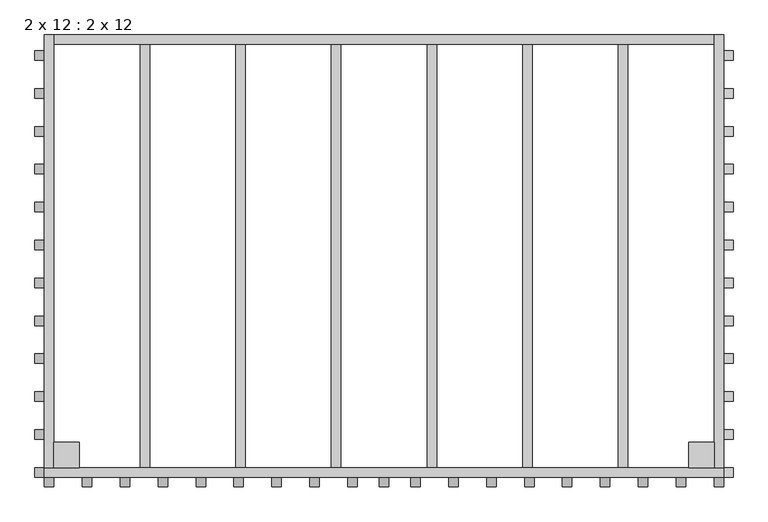
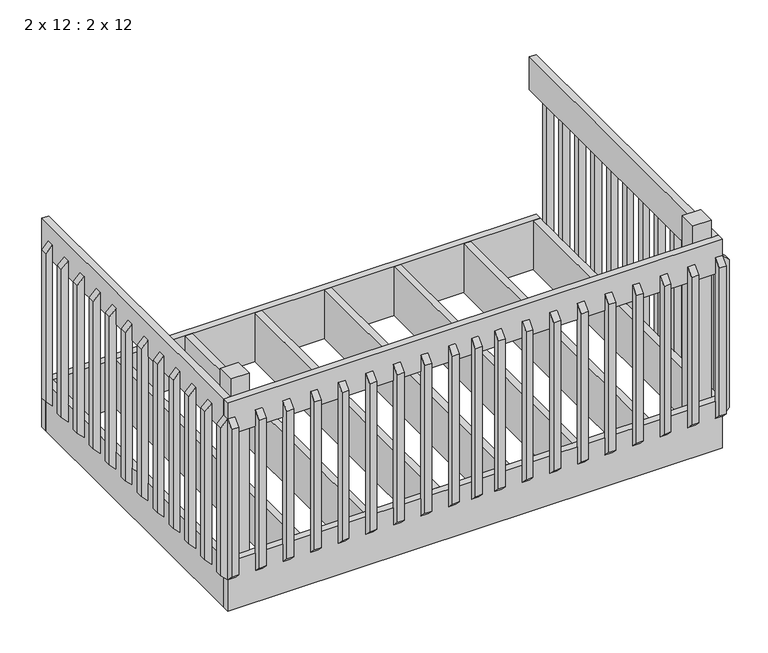
"""IFC4 building model written with IfcOpenShell, lengths in millimetres: proxy geometry, 2 x 12 : 2 x 12."""

from ifc_helpers import new_model, si_unit, frame, origin, place, context, project, spatial, polyline, outline, extrude, source, transform, mapped, element, save


def proxy_2_x_12_2_x_12_a4ed22fe(model_context):
    return source(origin(), model_context, "Body", "SweptSolid", [
        extrude(outline(polyline([(-24301.8830088, 3282.95), (-24339.9830088, 3321.05), (-24339.9830088, 4184.65), (-24301.8830088, 4222.75), (-24301.8830088, 3282.95)])), frame((31168.6652986, 0.0, 0.0), z_axis=(1.0, 0.0, 0.0), x_axis=(0.0, 1.0, 0.0)), (0.0, 0.0, 1.0), 38.1),
        extrude(outline(polyline([(-24301.8830088, 3282.95), (-24339.9830088, 3321.05), (-24339.9830088, 4184.65), (-24301.8830088, 4222.75), (-24301.8830088, 3282.95)])), frame((31295.6652986, 0.0, 0.0), z_axis=(1.0, 0.0, 0.0), x_axis=(0.0, 1.0, 0.0)), (0.0, 0.0, 1.0), 38.1),
        extrude(outline(polyline([(-24301.8830088, 3282.95), (-24339.9830088, 3321.05), (-24339.9830088, 4184.65), (-24301.8830088, 4222.75), (-24301.8830088, 3282.95)])), frame((31448.0652986, 0.0, 0.0), z_axis=(1.0, 0.0, 0.0), x_axis=(0.0, 1.0, 0.0)), (0.0, 0.0, 1.0), 38.1),
        extrude(outline(polyline([(-24301.8830088, 3282.95), (-24339.9830088, 3321.05), (-24339.9830088, 4184.65), (-24301.8830088, 4222.75), (-24301.8830088, 3282.95)])), frame((31600.4652986, 0.0, 0.0), z_axis=(1.0, 0.0, 0.0), x_axis=(0.0, 1.0, 0.0)), (0.0, 0.0, 1.0), 38.1),
        extrude(outline(polyline([(-24301.8830088, 3282.95), (-24339.9830088, 3321.05), (-24339.9830088, 4184.65), (-24301.8830088, 4222.75), (-24301.8830088, 3282.95)])), frame((31752.8652986, 0.0, 0.0), z_axis=(1.0, 0.0, 0.0), x_axis=(0.0, 1.0, 0.0)), (0.0, 0.0, 1.0), 38.1),
        extrude(outline(polyline([(-24301.8830088, 3282.95), (-24339.9830088, 3321.05), (-24339.9830088, 4184.65), (-24301.8830088, 4222.75), (-24301.8830088, 3282.95)])), frame((31905.2652986, 0.0, 0.0), z_axis=(1.0, 0.0, 0.0), x_axis=(0.0, 1.0, 0.0)), (0.0, 0.0, 1.0), 38.1),
        extrude(outline(polyline([(-24301.8830088, 3282.95), (-24339.9830088, 3321.05), (-24339.9830088, 4184.65), (-24301.8830088, 4222.75), (-24301.8830088, 3282.95)])), frame((32057.6652986, 0.0, 0.0), z_axis=(1.0, 0.0, 0.0), x_axis=(0.0, 1.0, 0.0)), (0.0, 0.0, 1.0), 38.1),
        extrude(outline(polyline([(-24301.8830088, 3282.95), (-24339.9830088, 3321.05), (-24339.9830088, 4184.65), (-24301.8830088, 4222.75), (-24301.8830088, 3282.95)])), frame((32210.0652986, 0.0, 0.0), z_axis=(1.0, 0.0, 0.0), x_axis=(0.0, 1.0, 0.0)), (0.0, 0.0, 1.0), 38.1),
        extrude(outline(polyline([(-24301.8830088, 3282.95), (-24339.9830088, 3321.05), (-24339.9830088, 4184.65), (-24301.8830088, 4222.75), (-24301.8830088, 3282.95)])), frame((32362.4652986, 0.0, 0.0), z_axis=(1.0, 0.0, 0.0), x_axis=(0.0, 1.0, 0.0)), (0.0, 0.0, 1.0), 38.1),
        extrude(outline(polyline([(-24301.8830088, 3282.95), (-24339.9830088, 3321.05), (-24339.9830088, 4184.65), (-24301.8830088, 4222.75), (-24301.8830088, 3282.95)])), frame((32514.8652986, 0.0, 0.0), z_axis=(1.0, 0.0, 0.0), x_axis=(0.0, 1.0, 0.0)), (0.0, 0.0, 1.0), 38.1),
        extrude(outline(polyline([(-24301.8830088, 3282.95), (-24339.9830088, 3321.05), (-24339.9830088, 4184.65), (-24301.8830088, 4222.75), (-24301.8830088, 3282.95)])), frame((29822.4652986, 0.0, 0.0), z_axis=(1.0, 0.0, 0.0), x_axis=(0.0, 1.0, 0.0)), (0.0, 0.0, 1.0), 38.1),
        extrude(outline(polyline([(-24301.8830088, 3282.95), (-24339.9830088, 3321.05), (-24339.9830088, 4184.65), (-24301.8830088, 4222.75), (-24301.8830088, 3282.95)])), frame((29974.8652986, 0.0, 0.0), z_axis=(1.0, 0.0, 0.0), x_axis=(0.0, 1.0, 0.0)), (0.0, 0.0, 1.0), 38.1),
        extrude(outline(polyline([(-24301.8830088, 3282.95), (-24339.9830088, 3321.05), (-24339.9830088, 4184.65), (-24301.8830088, 4222.75), (-24301.8830088, 3282.95)])), frame((30127.2652986, 0.0, 0.0), z_axis=(1.0, 0.0, 0.0), x_axis=(0.0, 1.0, 0.0)), (0.0, 0.0, 1.0), 38.1),
        extrude(outline(polyline([(-24301.8830088, 3282.95), (-24339.9830088, 3321.05), (-24339.9830088, 4184.65), (-24301.8830088, 4222.75), (-24301.8830088, 3282.95)])), frame((30279.6652986, 0.0, 0.0), z_axis=(1.0, 0.0, 0.0), x_axis=(0.0, 1.0, 0.0)), (0.0, 0.0, 1.0), 38.1),
        extrude(outline(polyline([(-24301.8830088, 3282.95), (-24339.9830088, 3321.05), (-24339.9830088, 4184.65), (-24301.8830088, 4222.75), (-24301.8830088, 3282.95)])), frame((30432.0652986, 0.0, 0.0), z_axis=(1.0, 0.0, 0.0), x_axis=(0.0, 1.0, 0.0)), (0.0, 0.0, 1.0), 38.1),
        extrude(outline(polyline([(-24301.8830088, 3282.95), (-24339.9830088, 3321.05), (-24339.9830088, 4184.65), (-24301.8830088, 4222.75), (-24301.8830088, 3282.95)])), frame((30584.4652986, 0.0, 0.0), z_axis=(1.0, 0.0, 0.0), x_axis=(0.0, 1.0, 0.0)), (0.0, 0.0, 1.0), 38.1),
        extrude(outline(polyline([(-24301.8830088, 3282.95), (-24339.9830088, 3321.05), (-24339.9830088, 4184.65), (-24301.8830088, 4222.75), (-24301.8830088, 3282.95)])), frame((30736.8652986, 0.0, 0.0), z_axis=(1.0, 0.0, 0.0), x_axis=(0.0, 1.0, 0.0)), (0.0, 0.0, 1.0), 38.1),
        extrude(outline(polyline([(-24301.8830088, 3282.95), (-24339.9830088, 3321.05), (-24339.9830088, 4184.65), (-24301.8830088, 4222.75), (-24301.8830088, 3282.95)])), frame((30889.2652986, 0.0, 0.0), z_axis=(1.0, 0.0, 0.0), x_axis=(0.0, 1.0, 0.0)), (0.0, 0.0, 1.0), 38.1),
        extrude(outline(polyline([(-24301.8830088, 3282.95), (-24339.9830088, 3321.05), (-24339.9830088, 4184.65), (-24301.8830088, 4222.75), (-24301.8830088, 3282.95)])), frame((31041.6652986, 0.0, 0.0), z_axis=(1.0, 0.0, 0.0), x_axis=(0.0, 1.0, 0.0)), (0.0, 0.0, 1.0), 38.1),
        extrude(outline(polyline([(3282.95, 29822.4652986), (4222.75, 29822.4652986), (4184.65, 29784.3652986), (3321.05, 29784.3652986), (3282.95, 29822.4652986)])), frame((0.0, -22625.4830088, 0.0), z_axis=(0.0, 1.0, 0.0), x_axis=(0.0, 0.0, 1.0)), (0.0, 0.0, 1.0), 38.1),
        extrude(outline(polyline([(3282.95, 29822.4652986), (4222.75, 29822.4652986), (4184.65, 29784.3652986), (3321.05, 29784.3652986), (3282.95, 29822.4652986)])), frame((0.0, -22777.8830088, 0.0), z_axis=(0.0, 1.0, 0.0), x_axis=(0.0, 0.0, 1.0)), (0.0, 0.0, 1.0), 38.1),
        extrude(outline(polyline([(3282.95, 29822.4652986), (4222.75, 29822.4652986), (4184.65, 29784.3652986), (3321.05, 29784.3652986), (3282.95, 29822.4652986)])), frame((0.0, -22930.2830088, 0.0), z_axis=(0.0, 1.0, 0.0), x_axis=(0.0, 0.0, 1.0)), (0.0, 0.0, 1.0), 38.1),
        extrude(outline(polyline([(3282.95, 29822.4652986), (4222.75, 29822.4652986), (4184.65, 29784.3652986), (3321.05, 29784.3652986), (3282.95, 29822.4652986)])), frame((0.0, -23082.6830088, 0.0), z_axis=(0.0, 1.0, 0.0), x_axis=(0.0, 0.0, 1.0)), (0.0, 0.0, 1.0), 38.1),
        extrude(outline(polyline([(3282.95, 29822.4652986), (4222.75, 29822.4652986), (4184.65, 29784.3652986), (3321.05, 29784.3652986), (3282.95, 29822.4652986)])), frame((0.0, -23235.0830088, 0.0), z_axis=(0.0, 1.0, 0.0), x_axis=(0.0, 0.0, 1.0)), (0.0, 0.0, 1.0), 38.1),
        extrude(outline(polyline([(3282.95, 29822.4652986), (4222.75, 29822.4652986), (4184.65, 29784.3652986), (3321.05, 29784.3652986), (3282.95, 29822.4652986)])), frame((0.0, -23387.4830088, 0.0), z_axis=(0.0, 1.0, 0.0), x_axis=(0.0, 0.0, 1.0)), (0.0, 0.0, 1.0), 38.1),
        extrude(outline(polyline([(3282.95, 29822.4652986), (4222.75, 29822.4652986), (4184.65, 29784.3652986), (3321.05, 29784.3652986), (3282.95, 29822.4652986)])), frame((0.0, -23539.8830088, 0.0), z_axis=(0.0, 1.0, 0.0), x_axis=(0.0, 0.0, 1.0)), (0.0, 0.0, 1.0), 38.1),
        extrude(outline(polyline([(3282.95, 29822.4652986), (4222.75, 29822.4652986), (4184.65, 29784.3652986), (3321.05, 29784.3652986), (3282.95, 29822.4652986)])), frame((0.0, -23692.2830088, 0.0), z_axis=(0.0, 1.0, 0.0), x_axis=(0.0, 0.0, 1.0)), (0.0, 0.0, 1.0), 38.1),
        extrude(outline(polyline([(3282.95, 29822.4652986), (4222.75, 29822.4652986), (4184.65, 29784.3652986), (3321.05, 29784.3652986), (3282.95, 29822.4652986)])), frame((0.0, -23844.6830088, 0.0), z_axis=(0.0, 1.0, 0.0), x_axis=(0.0, 0.0, 1.0)), (0.0, 0.0, 1.0), 38.1),
        extrude(outline(polyline([(3282.95, 29822.4652986), (4222.75, 29822.4652986), (4184.65, 29784.3652986), (3321.05, 29784.3652986), (3282.95, 29822.4652986)])), frame((0.0, -23997.0830088, 0.0), z_axis=(0.0, 1.0, 0.0), x_axis=(0.0, 0.0, 1.0)), (0.0, 0.0, 1.0), 38.1),
        extrude(outline(polyline([(3282.95, 29822.4652986), (4222.75, 29822.4652986), (4184.65, 29784.3652986), (3321.05, 29784.3652986), (3282.95, 29822.4652986)])), frame((0.0, -24149.4830088, 0.0), z_axis=(0.0, 1.0, 0.0), x_axis=(0.0, 0.0, 1.0)), (0.0, 0.0, 1.0), 38.1),
        extrude(outline(polyline([(3282.95, 29822.4652986), (4222.75, 29822.4652986), (4184.65, 29784.3652986), (3321.05, 29784.3652986), (3282.95, 29822.4652986)])), frame((0.0, -24301.8830088, 0.0), z_axis=(0.0, 1.0, 0.0), x_axis=(0.0, 0.0, 1.0)), (0.0, 0.0, 1.0), 38.1),
        extrude(outline(polyline([(3282.95, 32552.9652986), (3321.05, 32591.0652986), (4184.65, 32591.0652986), (4222.75, 32552.9652986), (3282.95, 32552.9652986)])), frame((0.0, -22625.4830088, 0.0), z_axis=(0.0, 1.0, 0.0), x_axis=(0.0, 0.0, 1.0)), (0.0, 0.0, 1.0), 38.1),
        extrude(outline(polyline([(3282.95, 32552.9652986), (3321.05, 32591.0652986), (4184.65, 32591.0652986), (4222.75, 32552.9652986), (3282.95, 32552.9652986)])), frame((0.0, -22777.8830088, 0.0), z_axis=(0.0, 1.0, 0.0), x_axis=(0.0, 0.0, 1.0)), (0.0, 0.0, 1.0), 38.1),
        extrude(outline(polyline([(3282.95, 32552.9652986), (3321.05, 32591.0652986), (4184.65, 32591.0652986), (4222.75, 32552.9652986), (3282.95, 32552.9652986)])), frame((0.0, -22930.2830088, 0.0), z_axis=(0.0, 1.0, 0.0), x_axis=(0.0, 0.0, 1.0)), (0.0, 0.0, 1.0), 38.1),
        extrude(outline(polyline([(3282.95, 32552.9652986), (3321.05, 32591.0652986), (4184.65, 32591.0652986), (4222.75, 32552.9652986), (3282.95, 32552.9652986)])), frame((0.0, -23082.6830088, 0.0), z_axis=(0.0, 1.0, 0.0), x_axis=(0.0, 0.0, 1.0)), (0.0, 0.0, 1.0), 38.1),
        extrude(outline(polyline([(3282.95, 32552.9652986), (3321.05, 32591.0652986), (4184.65, 32591.0652986), (4222.75, 32552.9652986), (3282.95, 32552.9652986)])), frame((0.0, -23235.0830088, 0.0), z_axis=(0.0, 1.0, 0.0), x_axis=(0.0, 0.0, 1.0)), (0.0, 0.0, 1.0), 38.1),
        extrude(outline(polyline([(3282.95, 32552.9652986), (3321.05, 32591.0652986), (4184.65, 32591.0652986), (4222.75, 32552.9652986), (3282.95, 32552.9652986)])), frame((0.0, -23387.4830088, 0.0), z_axis=(0.0, 1.0, 0.0), x_axis=(0.0, 0.0, 1.0)), (0.0, 0.0, 1.0), 38.1),
        extrude(outline(polyline([(3282.95, 32552.9652986), (3321.05, 32591.0652986), (4184.65, 32591.0652986), (4222.75, 32552.9652986), (3282.95, 32552.9652986)])), frame((0.0, -23539.8830088, 0.0), z_axis=(0.0, 1.0, 0.0), x_axis=(0.0, 0.0, 1.0)), (0.0, 0.0, 1.0), 38.1),
        extrude(outline(polyline([(3282.95, 32552.9652986), (3321.05, 32591.0652986), (4184.65, 32591.0652986), (4222.75, 32552.9652986), (3282.95, 32552.9652986)])), frame((0.0, -23692.2830088, 0.0), z_axis=(0.0, 1.0, 0.0), x_axis=(0.0, 0.0, 1.0)), (0.0, 0.0, 1.0), 38.1),
        extrude(outline(polyline([(3282.95, 32552.9652986), (3321.05, 32591.0652986), (4184.65, 32591.0652986), (4222.75, 32552.9652986), (3282.95, 32552.9652986)])), frame((0.0, -23844.6830088, 0.0), z_axis=(0.0, 1.0, 0.0), x_axis=(0.0, 0.0, 1.0)), (0.0, 0.0, 1.0), 38.1),
        extrude(outline(polyline([(3282.95, 32552.9652986), (3321.05, 32591.0652986), (4184.65, 32591.0652986), (4222.75, 32552.9652986), (3282.95, 32552.9652986)])), frame((0.0, -23997.0830088, 0.0), z_axis=(0.0, 1.0, 0.0), x_axis=(0.0, 0.0, 1.0)), (0.0, 0.0, 1.0), 38.1),
        extrude(outline(polyline([(3282.95, 32552.9652986), (3321.05, 32591.0652986), (4184.65, 32591.0652986), (4222.75, 32552.9652986), (3282.95, 32552.9652986)])), frame((0.0, -24149.4830088, 0.0), z_axis=(0.0, 1.0, 0.0), x_axis=(0.0, 0.0, 1.0)), (0.0, 0.0, 1.0), 38.1),
        extrude(outline(polyline([(3282.95, 32552.9652986), (3321.05, 32591.0652986), (4184.65, 32591.0652986), (4222.75, 32552.9652986), (3282.95, 32552.9652986)])), frame((0.0, -24301.8830088, 0.0), z_axis=(0.0, 1.0, 0.0), x_axis=(0.0, 0.0, 1.0)), (0.0, 0.0, 1.0), 38.1),
        extrude(outline(polyline([(29860.5652986, -24263.7830088), (29822.4652986, -24263.7830088), (29822.4652986, -22523.8830088), (29860.5652986, -22523.8830088), (29860.5652986, -24263.7830088)])), frame((0.0, 0.0, 4127.5), z_axis=(0.0, 0.0, 1.0), x_axis=(1.0, 0.0, 0.0)), (0.0, 0.0, 1.0), 190.5),
        extrude(outline(polyline([(32552.9652986, -24263.7830088), (32514.8652986, -24263.7830088), (32514.8652986, -22523.8830088), (32552.9652986, -22523.8830088), (32552.9652986, -24263.7830088)])), frame((0.0, 0.0, 4127.5), z_axis=(0.0, 0.0, 1.0), x_axis=(1.0, 0.0, 0.0)), (0.0, 0.0, 1.0), 190.5),
        extrude(outline(polyline([(32552.9652986, -24263.7830088), (32552.9652986, -24301.8830088), (29822.4652986, -24301.8830088), (29822.4652986, -24263.7830088), (32552.9652986, -24263.7830088)])), frame((0.0, 0.0, 4127.5), z_axis=(0.0, 0.0, 1.0), x_axis=(1.0, 0.0, 0.0)), (0.0, 0.0, 1.0), 190.5),
        extrude(outline(polyline([(32514.8652986, -24162.1830088), (32514.8652986, -24263.7830088), (32413.2652986, -24263.7830088), (32413.2652986, -24162.1830088), (32514.8652986, -24162.1830088)])), frame((0.0, 0.0, 3098.8), z_axis=(0.0, 0.0, 1.0), x_axis=(1.0, 0.0, 0.0)), (0.0, 0.0, 1.0), 1320.8),
        extrude(outline(polyline([(29962.1652986, -24162.1830088), (29962.1652986, -24263.7830088), (29860.5652986, -24263.7830088), (29860.5652986, -24162.1830088), (29962.1652986, -24162.1830088)])), frame((0.0, 0.0, 3098.8), z_axis=(0.0, 0.0, 1.0), x_axis=(1.0, 0.0, 0.0)), (0.0, 0.0, 1.0), 1320.8),
        extrude(outline(polyline([(32552.9652986, -22523.8830088), (32552.9652986, -22561.9830088), (29822.4652986, -22561.9830088), (29822.4652986, -22523.8830088), (32552.9652986, -22523.8830088)])), frame((0.0, 0.0, 3098.8), z_axis=(0.0, 0.0, 1.0), x_axis=(1.0, 0.0, 0.0)), (0.0, 0.0, 1.0), 285.75),
        extrude(outline(polyline([(32552.9652986, -24263.7830088), (32552.9652986, -24301.8830088), (29822.4652986, -24301.8830088), (29822.4652986, -24263.7830088), (32552.9652986, -24263.7830088)])), frame((0.0, 0.0, 3098.8), z_axis=(0.0, 0.0, 1.0), x_axis=(1.0, 0.0, 0.0)), (0.0, 0.0, 1.0), 285.75),
        extrude(outline(polyline([(32168.3367272, -24263.7830088), (32130.2367272, -24263.7830088), (32130.2367272, -22561.9830088), (32168.3367272, -22561.9830088), (32168.3367272, -24263.7830088)])), frame((0.0, 0.0, 3098.8), z_axis=(0.0, 0.0, 1.0), x_axis=(1.0, 0.0, 0.0)), (0.0, 0.0, 1.0), 285.75),
        extrude(outline(polyline([(31783.7081558, -24263.7830088), (31745.6081558, -24263.7830088), (31745.6081558, -22561.9830088), (31783.7081558, -22561.9830088), (31783.7081558, -24263.7830088)])), frame((0.0, 0.0, 3098.8), z_axis=(0.0, 0.0, 1.0), x_axis=(1.0, 0.0, 0.0)), (0.0, 0.0, 1.0), 285.75),
        extrude(outline(polyline([(31399.0795843, -24263.7830088), (31360.9795843, -24263.7830088), (31360.9795843, -22561.9830088), (31399.0795843, -22561.9830088), (31399.0795843, -24263.7830088)])), frame((0.0, 0.0, 3098.8), z_axis=(0.0, 0.0, 1.0), x_axis=(1.0, 0.0, 0.0)), (0.0, 0.0, 1.0), 285.75),
        extrude(outline(polyline([(31014.4510129, -24263.7830088), (30976.3510129, -24263.7830088), (30976.3510129, -22561.9830088), (31014.4510129, -22561.9830088), (31014.4510129, -24263.7830088)])), frame((0.0, 0.0, 3098.8), z_axis=(0.0, 0.0, 1.0), x_axis=(1.0, 0.0, 0.0)), (0.0, 0.0, 1.0), 285.75),
        extrude(outline(polyline([(30629.8224415, -24263.7830088), (30591.7224415, -24263.7830088), (30591.7224415, -22561.9830088), (30629.8224415, -22561.9830088), (30629.8224415, -24263.7830088)])), frame((0.0, 0.0, 3098.8), z_axis=(0.0, 0.0, 1.0), x_axis=(1.0, 0.0, 0.0)), (0.0, 0.0, 1.0), 285.75),
        extrude(outline(polyline([(30245.1938701, -24263.7830088), (30207.0938701, -24263.7830088), (30207.0938701, -22561.9830088), (30245.1938701, -22561.9830088), (30245.1938701, -24263.7830088)])), frame((0.0, 0.0, 3098.8), z_axis=(0.0, 0.0, 1.0), x_axis=(1.0, 0.0, 0.0)), (0.0, 0.0, 1.0), 285.75),
        extrude(outline(polyline([(32552.9652986, -24263.7830088), (32514.8652986, -24263.7830088), (32514.8652986, -22561.9830088), (32552.9652986, -22561.9830088), (32552.9652986, -24263.7830088)])), frame((0.0, 0.0, 3098.8), z_axis=(0.0, 0.0, 1.0), x_axis=(1.0, 0.0, 0.0)), (0.0, 0.0, 1.0), 285.75),
        extrude(outline(polyline([(29860.5652986, -24263.7830088), (29822.4652986, -24263.7830088), (29822.4652986, -22561.9830088), (29860.5652986, -22561.9830088), (29860.5652986, -24263.7830088)])), frame((0.0, 0.0, 3098.8), z_axis=(0.0, 0.0, 1.0), x_axis=(1.0, 0.0, 0.0)), (0.0, 0.0, 1.0), 285.75),
    ])


if __name__ == "__main__":
    model = new_model("IFC4")
    model_context = context("Model", 3, world=origin())
    ifc_project = project(units=[si_unit("LENGTHUNIT", "METRE", prefix="MILLI")], contexts=[model_context])
    site = spatial("IfcSite", under=ifc_project)
    building = spatial("IfcBuilding", under=site)
    placement = place(None, origin())
    proxy_2_x_12_2_x_12_shape = proxy_2_x_12_2_x_12_a4ed22fe(model_context)
    element("IfcBuildingElementProxy", 1, Name="2 x 12 : 2 x 12", ObjectType="2 x 12 : 2 x 12", at=placement, inside=building, context=model_context, shape_type="MappedRepresentation", body=[
        mapped(proxy_2_x_12_2_x_12_shape, transform((0.0, 0.0, 0.0), x_axis=(1.0, 0.0, 0.0), y_axis=(0.0, 1.0, 0.0), z_axis=(0.0, 0.0, 1.0))),
    ])
    save(model, "model.ifc")

# Revit data of these elements
# Element 1 (IfcBuildingElementProxy, "2 x 12 : 2 x 12")
#   Materials on its faces: "1.5\" X 1.5\" WOOD RAIL DECK STUDS", "2 X 12 WOOD DECK STUDS", "2 X 8 WOOD DECK STUDS", "4\" X 4\" CORNER RAIL POST"
# Materials
#   "1.5\" X 1.5\" WOOD RAIL DECK STUDS": class "Wood", colour RGB 144 113 62, transparency 0, Description = "Pinus Echinata", Cost = 0
#   "2 X 12 WOOD DECK STUDS": class "Wood", colour RGB 144 113 62, transparency 0, Description = "Pinus Echinata", Cost = 0
#   "2 X 8 WOOD DECK STUDS": class "Wood", colour RGB 144 113 62, transparency 0, Description = "Pinus Echinata", Cost = 0
#   "4\" X 4\" CORNER RAIL POST": class "Wood", colour RGB 144 113 62, transparency 0, Description = "Pinus Echinata", Cost = 0
